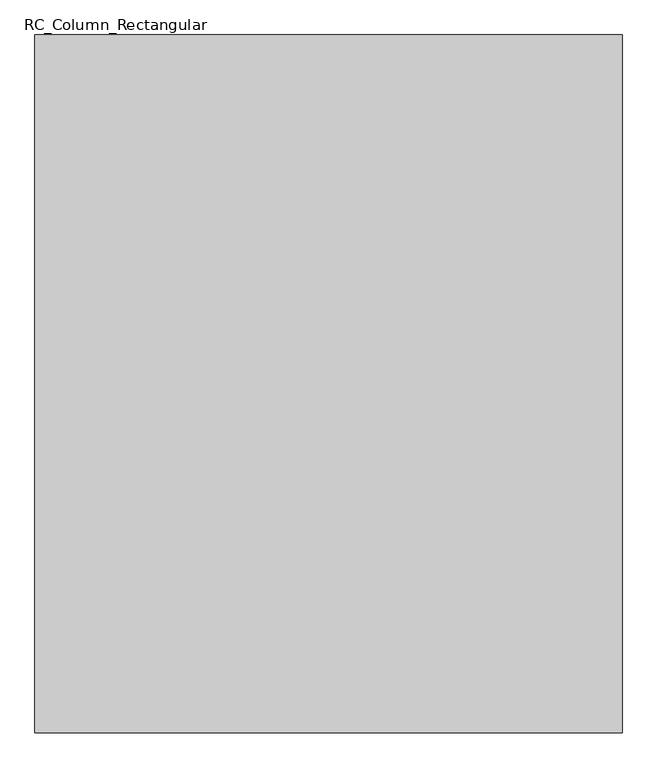
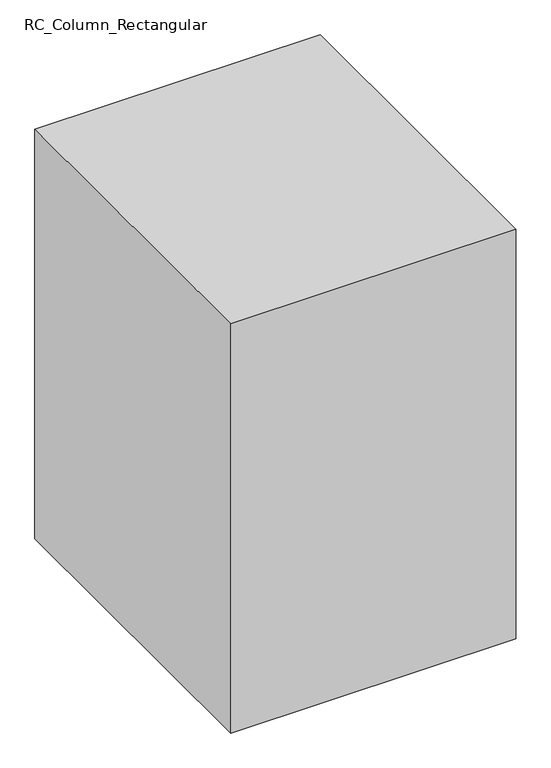
"""IFC4 building model written with IfcOpenShell, lengths in millimetres: column geometry, RC_Column_Rectangular : H_SC_AR_S15_AG Column_900x1070_C1."""

from ifc_helpers import new_model, si_unit, frame, origin, place, context, project, spatial, polyline, outline, extrude, source, transform, mapped, element, save


def rc_column_rectangular_1dd1414b(model_context):
    return source(origin(), model_context, "Body", "SweptSolid", [
        extrude(outline(polyline([(450.0, 535.0), (450.0, -535.0), (-450.0, -535.0), (-450.0, 535.0), (450.0, 535.0)])), frame((0.0, 0.0, 4799.9618634), z_axis=(0.0, 0.0, 1.0), x_axis=(1.0, 0.0, 0.0)), (0.0, 0.0, 1.0), 1365.0381366),
    ])


if __name__ == "__main__":
    model = new_model("IFC4")
    model_context = context("Model", 3, world=origin())
    ifc_project = project(units=[si_unit("LENGTHUNIT", "METRE", prefix="MILLI")], contexts=[model_context])
    site = spatial("IfcSite", under=ifc_project)
    building = spatial("IfcBuilding", under=site)
    placement = place(None, origin())
    rc_column_rectangular_shape = rc_column_rectangular_1dd1414b(model_context)
    element("IfcColumn", 1, ObjectType="RC_Column_Rectangular : H_SC_AR_S15_AG Column_900x1070_C1", at=placement, inside=building, context=model_context, shape_type="MappedRepresentation", body=[
        mapped(rc_column_rectangular_shape, transform((0.0, 0.0, 0.0), x_axis=(1.0, 0.0, 0.0), y_axis=(0.0, 1.0, 0.0), z_axis=(0.0, 0.0, 1.0))),
    ])
    save(model, "model.ifc")

# Revit data of these elements
# Type "RC_Column_Rectangular : H_SC_AR_S15_AG Column_900x1070_C1"
#   Type Comments = "CV-AG"
#   Type Mark = ""
#   Width = 900 mm
#   Length = 1070 mm
#   hec_material3 [instance default] = none
#   hec_material2 [instance default] = none
#   hec_material1 [instance default] = none
#   Structural Material [instance default] = none
#   Description = (empty or 0)
# Element 1 (IfcColumn, "RC_Column_Rectangular : H_SC_AR_S15_AG Column_900x1070_C1")
#   Structural Material = Concrete_f'c=28MPa(Cylender)
#   Materials on its faces: "Concrete_f'c=28MPa(Cylender)"
# Materials
#   "Concrete_f'c=28MPa(Cylender)": class "Concrete", colour RGB 176 176 176, transparency 0, Description = "Reinf. Conc.", Cost = 0, Image = Concrete.Cast-In-Place.Flat.Polished.Grey.jpg
